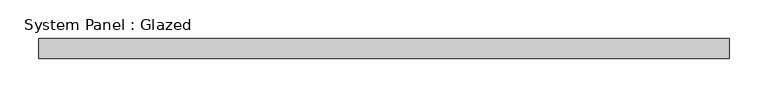
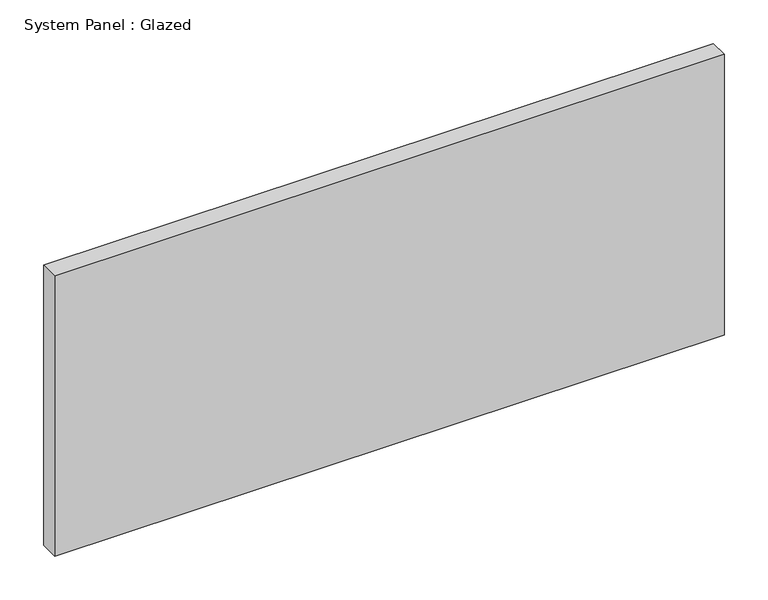
"""IFC4 building model written with IfcOpenShell, lengths in millimetres: plate geometry, System Panel : Glazed."""

from ifc_helpers import new_model, si_unit, origin, origin_with_axes, place, context, project, spatial, polyline, outline, extrude, source, transform, mapped, element, save


def system_panel_glazed_2014c690(model_context):
    return source(origin(), model_context, "Body", "SweptSolid", [
        extrude(outline(polyline([(444.4999998, -44.45), (-444.4999998, -44.45), (-444.4999998, -19.05), (444.4999998, -19.05), (444.4999998, -44.45)])), origin_with_axes(), (0.0, 0.0, 1.0), 393.7),
    ])


if __name__ == "__main__":
    model = new_model("IFC4")
    model_context = context("Model", 3, world=origin())
    ifc_project = project(units=[si_unit("LENGTHUNIT", "METRE", prefix="MILLI")], contexts=[model_context])
    site = spatial("IfcSite", under=ifc_project)
    building = spatial("IfcBuilding", under=site)
    placement = place(None, origin())
    system_panel_glazed_shape = system_panel_glazed_2014c690(model_context)
    element("IfcPlate", 1, ObjectType="System Panel : Glazed", at=placement, inside=building, context=model_context, shape_type="MappedRepresentation", body=[
        mapped(system_panel_glazed_shape, transform((0.0, 0.0, 0.0), x_axis=(1.0, 0.0, 0.0), y_axis=(0.0, 1.0, 0.0), z_axis=(0.0, 0.0, 1.0))),
    ])
    save(model, "model.ifc")

# Revit data of these elements
# Element 1 (IfcPlate, "System Panel : Glazed")
#   Materials on its faces: "Glass"
# Materials
#   "Glass": class "Glass", colour RGB 0 128 192, transparency 0.75
